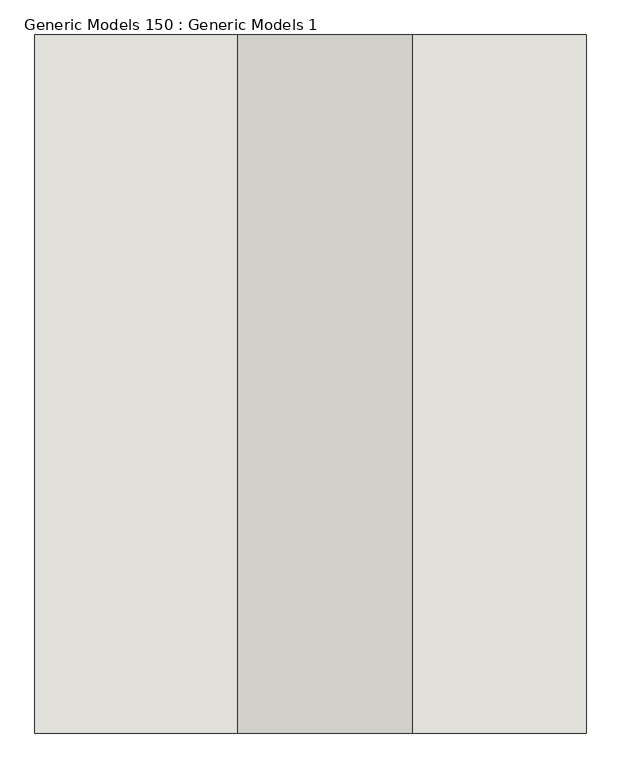
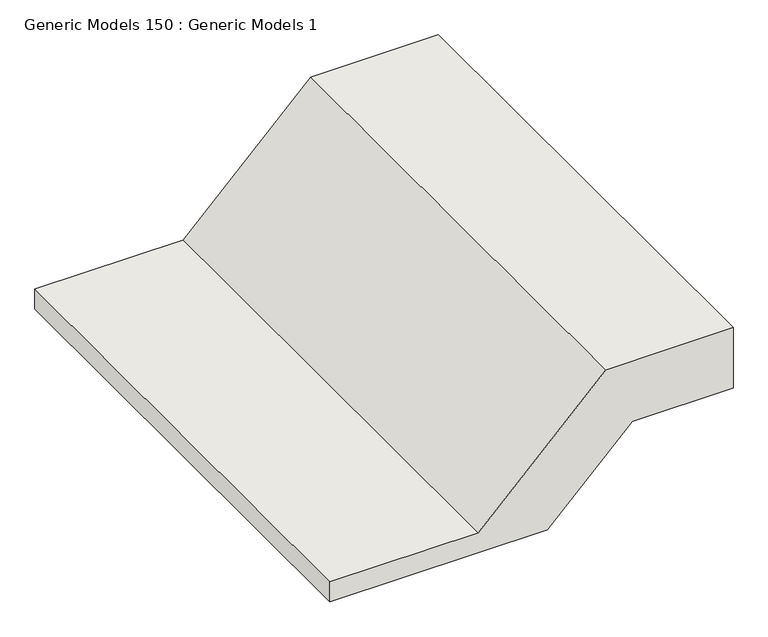
"""IFC4 building model written with IfcOpenShell, lengths in millimetres: wall geometry, Generic Models 150 : Generic Models 1."""

import ifcopenshell
import ifcopenshell.guid

model = None  # the IFC model being written
_history = None  # IfcOwnerHistory: only IFC2X3 demands one
_inside = {}  # id of a spatial element -> (the spatial element, [elements in it])
_under = {}  # id of a project, library or spatial element -> (it, [spatial elements below it])
_declared = {}  # id of a project -> (the project, [libraries it declares])
_typed = {}  # id of a type object -> (the type object, [elements of that type])
_made_of = {}  # id of a material, layer set ... -> (it, [elements and type objects made of it])


def new_model(schema):
    """Start an empty IFC model of exactly this schema.

    Asked for "IFC4X3", IfcOpenShell would pick the latest addendum, in which some entities
    have other attributes; the version numbers below select the first issue.
    IFC2X3 requires an IfcOwnerHistory on every rooted entity: one is made here for all.
    """
    global model, _history
    if schema == "IFC4X3":
        model = ifcopenshell.file(schema_version=(4, 3, 0, 0))
    else:
        model = ifcopenshell.file(schema=schema)
    _inside.clear()
    _under.clear()
    _declared.clear()
    _typed.clear()
    _made_of.clear()
    _history = None
    if model.schema == "IFC2X3":
        org = make("IfcOrganization", Name="unknown")
        user = make(
            "IfcPersonAndOrganization",
            ThePerson=make("IfcPerson", FamilyName="unknown"),
            TheOrganization=org,
        )
        app = make(
            "IfcApplication",
            ApplicationDeveloper=org,
            Version="unknown",
            ApplicationFullName="unknown",
            ApplicationIdentifier="unknown",
        )
        _history = make(
            "IfcOwnerHistory",
            OwningUser=user,
            OwningApplication=app,
            ChangeAction="ADDED",
            CreationDate=0,
        )
    return model


def make(cls, **values):
    """One entity of the class cls with the attributes given. An attribute that is None is left unset."""
    return model.create_entity(
        cls, **{name: value for name, value in values.items() if value is not None}
    )


def rooted(cls, **values):
    """An entity with a GlobalId (a new one), such as an element, a storey or a relation."""
    return make(cls, GlobalId=ifcopenshell.guid.new(), OwnerHistory=_history, **values)


def si_unit(unit_type, name, prefix=None):
    """IfcSIUnit, for example si_unit("LENGTHUNIT", "METRE", prefix="MILLI")."""
    return make("IfcSIUnit", UnitType=unit_type, Prefix=prefix, Name=name)


def assignment(units):
    """IfcUnitAssignment: the units of a project."""
    return None if units is None else make("IfcUnitAssignment", Units=units)


def point(xyz):
    """IfcCartesianPoint."""
    return None if xyz is None else make("IfcCartesianPoint", Coordinates=xyz)


def direction(xyz):
    """IfcDirection."""
    return None if xyz is None else make("IfcDirection", DirectionRatios=xyz)


def frame(location, z_axis=None, x_axis=None):
    """IfcAxis2Placement3D, a coordinate frame: its origin and axes. An axis left out is left unset."""
    return make(
        "IfcAxis2Placement3D",
        Location=point(location),
        Axis=direction(z_axis),
        RefDirection=direction(x_axis),
    )


def origin():
    """The frame at (0, 0, 0) with its axes left unset."""
    return frame((0.0, 0.0, 0.0))


def place(relative_to, where):
    """IfcLocalPlacement: puts the frame where relative to a parent placement (None: the world)."""
    return make(
        "IfcLocalPlacement", PlacementRelTo=relative_to, RelativePlacement=where
    )


def context(
    kind, dimensions, precision=None, world=None, true_north=None, identifier=None
):
    """IfcGeometricRepresentationContext, for example the 3D "Model" context."""
    return make(
        "IfcGeometricRepresentationContext",
        ContextIdentifier=identifier,
        ContextType=kind,
        CoordinateSpaceDimension=dimensions,
        Precision=precision,
        WorldCoordinateSystem=world,
        TrueNorth=true_north,
    )


def project(units=None, contexts=None):
    """IfcProject with its units and contexts."""
    return rooted(
        "IfcProject",
        Name="project",
        RepresentationContexts=contexts,
        UnitsInContext=assignment(units),
    )


def spatial(cls, under=None, at=None, **own):
    """A site, building, storey or space (cls), placed at a placement, below another one or the project."""
    s = rooted(cls, ObjectPlacement=at, **own)
    if under is not None:
        _under.setdefault(under.id(), (under, []))[1].append(s)
    return s


def polyline(points):
    """IfcPolyline through the points."""
    return make("IfcPolyline", Points=[point(p) for p in points])


def outline(outer, holes=None, kind="AREA"):
    """IfcArbitraryClosedProfileDef: a profile drawn as a closed curve; with holes, ...WithVoids."""
    if holes is None:
        return make("IfcArbitraryClosedProfileDef", ProfileType=kind, OuterCurve=outer)
    return make(
        "IfcArbitraryProfileDefWithVoids",
        ProfileType=kind,
        OuterCurve=outer,
        InnerCurves=holes,
    )


def extrude(swept, where, along, depth):
    """IfcExtrudedAreaSolid: the profile swept, set in the frame where, extruded along a direction by depth."""
    return make(
        "IfcExtrudedAreaSolid",
        SweptArea=swept,
        Position=where,
        ExtrudedDirection=direction(along),
        Depth=depth,
    )


def shape(context_of_items, identifier, shape_type, items):
    """IfcShapeRepresentation: the items that make up one representation, for example the "Body"."""
    return make(
        "IfcShapeRepresentation",
        ContextOfItems=context_of_items,
        RepresentationIdentifier=identifier,
        RepresentationType=shape_type,
        Items=items,
    )


def source(mapping_origin, context_of_items, identifier, shape_type, items):
    """IfcRepresentationMap: a shape defined once, which mapped items show again and again."""
    return make(
        "IfcRepresentationMap",
        MappingOrigin=mapping_origin,
        MappedRepresentation=shape(context_of_items, identifier, shape_type, items),
    )


def transform(
    local_origin,
    x_axis=None,
    y_axis=None,
    z_axis=None,
    scale=None,
    scale2=None,
    scale3=None,
    uniform=True,
):
    """IfcCartesianTransformationOperator3D, or its non-uniform kind. x_axis, y_axis, z_axis: its Axis1, 2, 3."""
    if uniform:
        return make(
            "IfcCartesianTransformationOperator3D",
            Axis1=direction(x_axis),
            Axis2=direction(y_axis),
            LocalOrigin=point(local_origin),
            Scale=scale,
            Axis3=direction(z_axis),
        )
    return make(
        "IfcCartesianTransformationOperator3DnonUniform",
        Axis1=direction(x_axis),
        Axis2=direction(y_axis),
        LocalOrigin=point(local_origin),
        Scale=scale,
        Axis3=direction(z_axis),
        Scale2=scale2,
        Scale3=scale3,
    )


def mapped(mapping_source, mapping_target):
    """IfcMappedItem: shows the shape of a source again, moved by a transform."""
    return make(
        "IfcMappedItem", MappingSource=mapping_source, MappingTarget=mapping_target
    )


def made_of(thing, what):
    """Note that an element or type object is made of a material, layer set ...; save() writes the relation."""
    if what is not None:
        _made_of.setdefault(what.id(), (what, []))[1].append(thing)
    return thing


def element(
    cls,
    number,
    at=None,
    inside=None,
    cuts=None,
    type_object=None,
    material=None,
    context=None,
    identifier="Body",
    shape_type=None,
    held_by="IfcProductDefinitionShape",
    body=None,
    shapes=None,
    **own,
):
    """One element of the class cls, such as IfcWall. Its Tag is "e" and its number.

    at: its placement. inside: the storey or other place that contains it. cuts: it is an
    opening in that element (IfcRelVoidsElement). A single representation is given by context,
    identifier, shape_type and body (its items); several are given by shapes. held_by: the class
    of the entity that holds the representations. save() writes the other relations.
    """
    e = rooted(cls, Tag="e%d" % number, ObjectPlacement=at, **own)
    if body is not None:
        shapes = [shape(context, identifier, shape_type, body)]
    if shapes is not None:
        e.Representation = make(held_by, Representations=shapes)
    if inside is not None:
        _inside.setdefault(inside.id(), (inside, []))[1].append(e)
    if cuts is not None:
        rooted(
            "IfcRelVoidsElement", RelatingBuildingElement=cuts, RelatedOpeningElement=e
        )
    if type_object is not None:
        _typed.setdefault(type_object.id(), (type_object, []))[1].append(e)
    return made_of(e, material)


def aggregate(whole, parts):
    """IfcRelAggregates: a whole, such as a stair, and the parts it consists of."""
    return rooted("IfcRelAggregates", RelatingObject=whole, RelatedObjects=parts)


def save(model, path):
    """Write the relations noted so far, then the file.

    IfcRelAggregates (storeys below a building ...), IfcRelContainedInSpatialStructure (elements
    in a storey), IfcRelDefinesByType, IfcRelAssociatesMaterial and IfcRelDeclares: one each for
    every whole, place, type object, material and project.
    """
    for whole, parts in _under.values():
        aggregate(whole, parts)
    for where, things in _inside.values():
        rooted(
            "IfcRelContainedInSpatialStructure",
            RelatedElements=things,
            RelatingStructure=where,
        )
    for kind, things in _typed.values():
        rooted("IfcRelDefinesByType", RelatedObjects=things, RelatingType=kind)
    for what, things in _made_of.values():
        rooted("IfcRelAssociatesMaterial", RelatedObjects=things, RelatingMaterial=what)
    for by, libraries in _declared.values():
        rooted("IfcRelDeclares", RelatingContext=by, RelatedDefinitions=libraries)
    model.write(path)


def generic_models_150_generic_models_1_b2c8ea2b(model_context):
    return source(origin(), model_context, "Body", "SweptSolid", [
        extrude(outline(polyline([(-310.1710164, 52787.3395874), (-157.7710164, 52787.3395874), (-157.7710164, 52483.7302124), (-462.5710164, 52178.9302124), (-462.5710164, 51824.8420742), (-513.3710164, 51824.8420742), (-513.3710164, 52343.6563593), (-310.1710164, 52546.8563593), (-310.1710164, 52787.3395874)])), frame((0.0, 0.0, 0.0), z_axis=(0.0, 1.0, 0.0), x_axis=(0.0, 0.0, 1.0)), (0.0, 0.0, 1.0), 1219.2),
    ])


if __name__ == "__main__":
    model = new_model("IFC4")
    model_context = context("Model", 3, world=origin())
    ifc_project = project(units=[si_unit("LENGTHUNIT", "METRE", prefix="MILLI")], contexts=[model_context])
    site = spatial("IfcSite", under=ifc_project)
    building = spatial("IfcBuilding", under=site)
    placement = place(None, origin())
    generic_models_150_generic_models_1_shape = generic_models_150_generic_models_1_b2c8ea2b(model_context)
    element("IfcWall", 1, ObjectType="Generic Models 150 : Generic Models 1", at=placement, inside=building, context=model_context, shape_type="MappedRepresentation", body=[
        mapped(generic_models_150_generic_models_1_shape, transform((0.0, 0.0, 0.0), x_axis=(1.0, 0.0, 0.0), y_axis=(0.0, 1.0, 0.0), z_axis=(0.0, 0.0, 1.0))),
    ])
    save(model, "model.ifc")

# Revit data of these elements
# Element 1 (IfcWall, "Generic Models 150 : Generic Models 1")
#   Materials on its faces: "6\" COMPACTED CRUSHED STONE"
# Materials
#   "6\" COMPACTED CRUSHED STONE": class "Generic", colour RGB 255 255 255, transparency 0, Cost = 0
